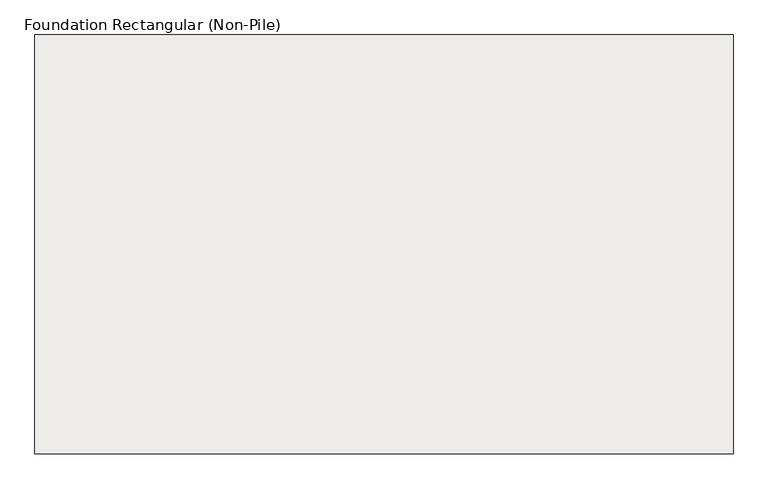
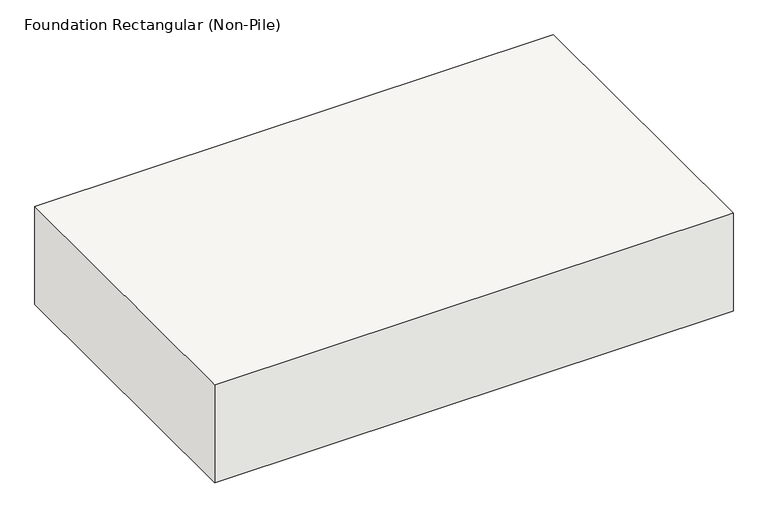
"""IFC4 building model written with IfcOpenShell, lengths in millimetres: slab geometry, Foundation Rectangular (Non-Pile) : H_SF_AR S18_Ret Fdn_F4 2500x1500x500."""

from ifc_helpers import new_model, si_unit, frame, origin, place, context, project, spatial, polyline, outline, extrude, source, transform, mapped, element, save


def foundation_rectangular_non_pile_907a7f09(model_context):
    return source(origin(), model_context, "Body", "SweptSolid", [
        extrude(outline(polyline([(1250.0, 750.0), (1250.0, -750.0), (-1250.0, -750.0), (-1250.0, 750.0), (1250.0, 750.0)])), frame((0.0, 0.0, -500.0), z_axis=(0.0, 0.0, 1.0), x_axis=(1.0, 0.0, 0.0)), (0.0, 0.0, 1.0), 500.0),
    ])


if __name__ == "__main__":
    model = new_model("IFC4")
    model_context = context("Model", 3, world=origin())
    ifc_project = project(units=[si_unit("LENGTHUNIT", "METRE", prefix="MILLI")], contexts=[model_context])
    site = spatial("IfcSite", under=ifc_project)
    building = spatial("IfcBuilding", under=site)
    placement = place(None, origin())
    foundation_rectangular_non_pile_shape = foundation_rectangular_non_pile_907a7f09(model_context)
    element("IfcSlab", 1, ObjectType="Foundation Rectangular (Non-Pile) : H_SF_AR S18_Ret Fdn_F4 2500x1500x500", at=placement, inside=building, context=model_context, shape_type="MappedRepresentation", body=[
        mapped(foundation_rectangular_non_pile_shape, transform((0.0, 0.0, 0.0), x_axis=(1.0, 0.0, 0.0), y_axis=(0.0, 1.0, 0.0), z_axis=(0.0, 0.0, 1.0))),
    ])
    save(model, "model.ifc")

# Revit data of these elements
# Type "Foundation Rectangular (Non-Pile) : H_SF_AR S18_Ret Fdn_F4 2500x1500x500"
#   Type Comments = "UG"
#   Type Mark = "F4"
#   Top bar = "D25@300"
#   Description = "UG Shallow Foundation"
#   Bottom bar = "D20@300"
#   H_Rebar Ratio = 0.12
#   Width = 2500 mm
#   Length = 1500 mm
#   Foundation Thickness = 500 mm
#   Structural Material [instance default] = none
#   Assembly Code = ""
# Element 1 (IfcSlab, "Foundation Rectangular (Non-Pile) : H_SF_AR S18_Ret Fdn_F4 2500x1500x500")
#   Materials on its faces: "00_Concrete_Reinf. Conc."
# Materials
#   "00_Concrete_Reinf. Conc.": class "Concrete", colour RGB 176 176 176, transparency 0, Description = "Reinf. Conc.", Cost = 0, Image = Concrete.Cast-In-Place.Flat.Polished.Grey.jpg
